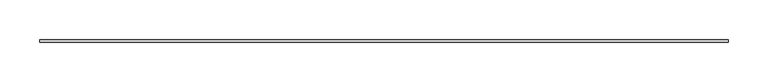
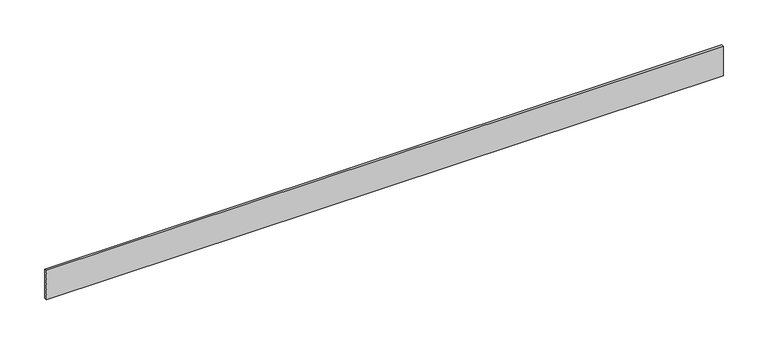
"""IFC4 building model written with IfcOpenShell, lengths in millimetres: proxy geometry, Generic Models 3:Generic Models 1:3:Generic Models 1:3 : Generic Models 3:Generic Models 1:300625:336034:Generic Models 1:3:Generic Models 1:3 : Generic Models 3:Generic Models 1:300625:336034 : Generic Models 3:Generic Models 1:3:Generic Models 1:3 : Generic Models 3:Generic Models 1:300625:336034:4 : Generic Models 3:Generic Models 1:3:Generic Models 1:3 : Generic Models 3:Generic Models 1:300625:336034:Generic Models 1:3:Generic Models 1:3 : Generic Models 3:Generic Models 1:300625:336034 : Generic Models 3:Generic Models 1:3:Generic Models 1:3 : Generic Models 3:Generic Models 1:300625:336034:301191."""

import ifcopenshell
import ifcopenshell.guid

model = None  # the IFC model being written
_history = None  # IfcOwnerHistory: only IFC2X3 demands one
_inside = {}  # id of a spatial element -> (the spatial element, [elements in it])
_under = {}  # id of a project, library or spatial element -> (it, [spatial elements below it])
_declared = {}  # id of a project -> (the project, [libraries it declares])
_typed = {}  # id of a type object -> (the type object, [elements of that type])
_made_of = {}  # id of a material, layer set ... -> (it, [elements and type objects made of it])


def new_model(schema):
    """Start an empty IFC model of exactly this schema.

    Asked for "IFC4X3", IfcOpenShell would pick the latest addendum, in which some entities
    have other attributes; the version numbers below select the first issue.
    IFC2X3 requires an IfcOwnerHistory on every rooted entity: one is made here for all.
    """
    global model, _history
    if schema == "IFC4X3":
        model = ifcopenshell.file(schema_version=(4, 3, 0, 0))
    else:
        model = ifcopenshell.file(schema=schema)
    _inside.clear()
    _under.clear()
    _declared.clear()
    _typed.clear()
    _made_of.clear()
    _history = None
    if model.schema == "IFC2X3":
        org = make("IfcOrganization", Name="unknown")
        user = make(
            "IfcPersonAndOrganization",
            ThePerson=make("IfcPerson", FamilyName="unknown"),
            TheOrganization=org,
        )
        app = make(
            "IfcApplication",
            ApplicationDeveloper=org,
            Version="unknown",
            ApplicationFullName="unknown",
            ApplicationIdentifier="unknown",
        )
        _history = make(
            "IfcOwnerHistory",
            OwningUser=user,
            OwningApplication=app,
            ChangeAction="ADDED",
            CreationDate=0,
        )
    return model


def make(cls, **values):
    """One entity of the class cls with the attributes given. An attribute that is None is left unset."""
    return model.create_entity(
        cls, **{name: value for name, value in values.items() if value is not None}
    )


def rooted(cls, **values):
    """An entity with a GlobalId (a new one), such as an element, a storey or a relation."""
    return make(cls, GlobalId=ifcopenshell.guid.new(), OwnerHistory=_history, **values)


def si_unit(unit_type, name, prefix=None):
    """IfcSIUnit, for example si_unit("LENGTHUNIT", "METRE", prefix="MILLI")."""
    return make("IfcSIUnit", UnitType=unit_type, Prefix=prefix, Name=name)


def assignment(units):
    """IfcUnitAssignment: the units of a project."""
    return None if units is None else make("IfcUnitAssignment", Units=units)


def point(xyz):
    """IfcCartesianPoint."""
    return None if xyz is None else make("IfcCartesianPoint", Coordinates=xyz)


def direction(xyz):
    """IfcDirection."""
    return None if xyz is None else make("IfcDirection", DirectionRatios=xyz)


def frame(location, z_axis=None, x_axis=None):
    """IfcAxis2Placement3D, a coordinate frame: its origin and axes. An axis left out is left unset."""
    return make(
        "IfcAxis2Placement3D",
        Location=point(location),
        Axis=direction(z_axis),
        RefDirection=direction(x_axis),
    )


def origin():
    """The frame at (0, 0, 0) with its axes left unset."""
    return frame((0.0, 0.0, 0.0))


def place(relative_to, where):
    """IfcLocalPlacement: puts the frame where relative to a parent placement (None: the world)."""
    return make(
        "IfcLocalPlacement", PlacementRelTo=relative_to, RelativePlacement=where
    )


def context(
    kind, dimensions, precision=None, world=None, true_north=None, identifier=None
):
    """IfcGeometricRepresentationContext, for example the 3D "Model" context."""
    return make(
        "IfcGeometricRepresentationContext",
        ContextIdentifier=identifier,
        ContextType=kind,
        CoordinateSpaceDimension=dimensions,
        Precision=precision,
        WorldCoordinateSystem=world,
        TrueNorth=true_north,
    )


def project(units=None, contexts=None):
    """IfcProject with its units and contexts."""
    return rooted(
        "IfcProject",
        Name="project",
        RepresentationContexts=contexts,
        UnitsInContext=assignment(units),
    )


def spatial(cls, under=None, at=None, **own):
    """A site, building, storey or space (cls), placed at a placement, below another one or the project."""
    s = rooted(cls, ObjectPlacement=at, **own)
    if under is not None:
        _under.setdefault(under.id(), (under, []))[1].append(s)
    return s


def polyline(points):
    """IfcPolyline through the points."""
    return make("IfcPolyline", Points=[point(p) for p in points])


def outline(outer, holes=None, kind="AREA"):
    """IfcArbitraryClosedProfileDef: a profile drawn as a closed curve; with holes, ...WithVoids."""
    if holes is None:
        return make("IfcArbitraryClosedProfileDef", ProfileType=kind, OuterCurve=outer)
    return make(
        "IfcArbitraryProfileDefWithVoids",
        ProfileType=kind,
        OuterCurve=outer,
        InnerCurves=holes,
    )


def extrude(swept, where, along, depth):
    """IfcExtrudedAreaSolid: the profile swept, set in the frame where, extruded along a direction by depth."""
    return make(
        "IfcExtrudedAreaSolid",
        SweptArea=swept,
        Position=where,
        ExtrudedDirection=direction(along),
        Depth=depth,
    )


def shape(context_of_items, identifier, shape_type, items):
    """IfcShapeRepresentation: the items that make up one representation, for example the "Body"."""
    return make(
        "IfcShapeRepresentation",
        ContextOfItems=context_of_items,
        RepresentationIdentifier=identifier,
        RepresentationType=shape_type,
        Items=items,
    )


def source(mapping_origin, context_of_items, identifier, shape_type, items):
    """IfcRepresentationMap: a shape defined once, which mapped items show again and again."""
    return make(
        "IfcRepresentationMap",
        MappingOrigin=mapping_origin,
        MappedRepresentation=shape(context_of_items, identifier, shape_type, items),
    )


def transform(
    local_origin,
    x_axis=None,
    y_axis=None,
    z_axis=None,
    scale=None,
    scale2=None,
    scale3=None,
    uniform=True,
):
    """IfcCartesianTransformationOperator3D, or its non-uniform kind. x_axis, y_axis, z_axis: its Axis1, 2, 3."""
    if uniform:
        return make(
            "IfcCartesianTransformationOperator3D",
            Axis1=direction(x_axis),
            Axis2=direction(y_axis),
            LocalOrigin=point(local_origin),
            Scale=scale,
            Axis3=direction(z_axis),
        )
    return make(
        "IfcCartesianTransformationOperator3DnonUniform",
        Axis1=direction(x_axis),
        Axis2=direction(y_axis),
        LocalOrigin=point(local_origin),
        Scale=scale,
        Axis3=direction(z_axis),
        Scale2=scale2,
        Scale3=scale3,
    )


def mapped(mapping_source, mapping_target):
    """IfcMappedItem: shows the shape of a source again, moved by a transform."""
    return make(
        "IfcMappedItem", MappingSource=mapping_source, MappingTarget=mapping_target
    )


def made_of(thing, what):
    """Note that an element or type object is made of a material, layer set ...; save() writes the relation."""
    if what is not None:
        _made_of.setdefault(what.id(), (what, []))[1].append(thing)
    return thing


def element(
    cls,
    number,
    at=None,
    inside=None,
    cuts=None,
    type_object=None,
    material=None,
    context=None,
    identifier="Body",
    shape_type=None,
    held_by="IfcProductDefinitionShape",
    body=None,
    shapes=None,
    **own,
):
    """One element of the class cls, such as IfcWall. Its Tag is "e" and its number.

    at: its placement. inside: the storey or other place that contains it. cuts: it is an
    opening in that element (IfcRelVoidsElement). A single representation is given by context,
    identifier, shape_type and body (its items); several are given by shapes. held_by: the class
    of the entity that holds the representations. save() writes the other relations.
    """
    e = rooted(cls, Tag="e%d" % number, ObjectPlacement=at, **own)
    if body is not None:
        shapes = [shape(context, identifier, shape_type, body)]
    if shapes is not None:
        e.Representation = make(held_by, Representations=shapes)
    if inside is not None:
        _inside.setdefault(inside.id(), (inside, []))[1].append(e)
    if cuts is not None:
        rooted(
            "IfcRelVoidsElement", RelatingBuildingElement=cuts, RelatedOpeningElement=e
        )
    if type_object is not None:
        _typed.setdefault(type_object.id(), (type_object, []))[1].append(e)
    return made_of(e, material)


def aggregate(whole, parts):
    """IfcRelAggregates: a whole, such as a stair, and the parts it consists of."""
    return rooted("IfcRelAggregates", RelatingObject=whole, RelatedObjects=parts)


def save(model, path):
    """Write the relations noted so far, then the file.

    IfcRelAggregates (storeys below a building ...), IfcRelContainedInSpatialStructure (elements
    in a storey), IfcRelDefinesByType, IfcRelAssociatesMaterial and IfcRelDeclares: one each for
    every whole, place, type object, material and project.
    """
    for whole, parts in _under.values():
        aggregate(whole, parts)
    for where, things in _inside.values():
        rooted(
            "IfcRelContainedInSpatialStructure",
            RelatedElements=things,
            RelatingStructure=where,
        )
    for kind, things in _typed.values():
        rooted("IfcRelDefinesByType", RelatedObjects=things, RelatingType=kind)
    for what, things in _made_of.values():
        rooted("IfcRelAssociatesMaterial", RelatedObjects=things, RelatingMaterial=what)
    for by, libraries in _declared.values():
        rooted("IfcRelDeclares", RelatingContext=by, RelatedDefinitions=libraries)
    model.write(path)


def generic_models_05a2607f(model_context):
    return source(origin(), model_context, "Body", "SweptSolid", [
        extrude(outline(polyline([(570395.4867239, -579000.6913841), (570395.4867239, -579003.8663841), (569527.1242239, -579003.8663841), (569527.1242239, -579000.6913841), (570395.4867239, -579000.6913841)])), frame((0.0, 0.0, 2446.5359375), z_axis=(0.0, 0.0, 1.0), x_axis=(1.0, 0.0, 0.0)), (0.0, 0.0, 1.0), 39.74694),
    ])


if __name__ == "__main__":
    model = new_model("IFC4")
    model_context = context("Model", 3, world=origin())
    ifc_project = project(units=[si_unit("LENGTHUNIT", "METRE", prefix="MILLI")], contexts=[model_context])
    site = spatial("IfcSite", under=ifc_project)
    building = spatial("IfcBuilding", under=site)
    placement = place(None, origin())
    generic_models_shape = generic_models_05a2607f(model_context)
    element("IfcBuildingElementProxy", 1, Name="Generic Models 3:Generic Models 1:3:Generic Models 1:3 : Generic Models 3:Generic Models 1:300625:336034:Generic Models 1:3:Generic Models 1:3 : Generic Models 3:Generic Models 1:300625:336034 : Generic Models 3:Generic Models 1:3:Generic Models 1:3 : Generic Models 3:Generic Models 1:300625:336034:4 : Generic Models 3:Generic Models 1:3:Generic Models 1:3 : Generic Models 3:Generic Models 1:300625:336034:Generic Models 1:3:Generic Models 1:3 : Generic Models 3:Generic Models 1:300625:336034 : Generic Models 3:Generic Models 1:3:Generic Models 1:3 : Generic Models 3:Generic Models 1:300625:336034:301191", ObjectType="Generic Models 3:Generic Models 1:3:Generic Models 1:3 : Generic Models 3:Generic Models 1:300625:336034:Generic Models 1:3:Generic Models 1:3 : Generic Models 3:Generic Models 1:300625:336034 : Generic Models 3:Generic Models 1:3:Generic Models 1:3 : Generic Models 3:Generic Models 1:300625:336034:4 : Generic Models 3:Generic Models 1:3:Generic Models 1:3 : Generic Models 3:Generic Models 1:300625:336034:Generic Models 1:3:Generic Models 1:3 : Generic Models 3:Generic Models 1:300625:336034 : Generic Models 3:Generic Models 1:3:Generic Models 1:3 : Generic Models 3:Generic Models 1:300625:336034:301191", at=placement, inside=building, context=model_context, shape_type="MappedRepresentation", body=[
        mapped(generic_models_shape, transform((0.0, 0.0, 0.0), x_axis=(1.0, 0.0, 0.0), y_axis=(0.0, 1.0, 0.0), z_axis=(0.0, 0.0, 1.0))),
    ])
    save(model, "model.ifc")

# Revit data of these elements
# Type "Generic Models 3:Generic Models 1:3:Generic Models 1:3 : Generic Models 3:Generic Models 1:300625:336034:Generic Models 1:3:Generic Models 1:3 : Generic Models 3:Generic Models 1:300625:336034 : Generic Models 3:Generic Models 1:3:Generic Models 1:3 : Generic Models 3:Generic Models 1:300625:336034:4 : Generic Models 3:Generic Models 1:3:Generic Models 1:3 : Generic Models 3:Generic Models 1:300625:336034:Generic Models 1:3:Generic Models 1:3 : Generic Models 3:Generic Models 1:300625:336034 : Generic Models 3:Generic Models 1:3:Generic Models 1:3 : Generic Models 3:Generic Models 1:300625:336034:301191"
#   NameOverride = "Generic Models 3:Generic Models 1:3:Generic Models 1:3 : Generic Models 3:Generic Models 1:300625:336034:Generic Models 1:3:Generic Models 1:3 : Generic Models 3:Generic Models 1:300625:336034 : Generic Models 3:Generic Models 1:3:Generic Models 1:3 : Generic Models 3:Generic Models 1:300625:336034:301191"
#   ObjectTypeOverride = "Generic Models 1:3:Generic Models 1:3 : Generic Models 3:Generic Models 1:300625:336034 : Generic Models 3:Generic Models 1:3:Generic Models 1:3 : Generic Models 3:Generic Models 1:300625:336034"
#   Reference = "Generic Models 1"
#   Tag = "301191"
# Element 1 (IfcBuildingElementProxy, "Generic Models 3:Generic Models 1:3:Generic Models 1:3 : Generic Models 3:Generic Models 1:300625:336034:Generic Models 1:3:Generic Models 1:3 : Generic Models 3:Generic Models 1:300625:336034 : Generic Models 3:Generic Models 1:3:Generic Models 1:3 : Generic Models 3:Generic Models 1:300625:336034:4 : Generic Models 3:Generic Models 1:3:Generic Models 1:3 : Generic Models 3:Generic Models 1:300625:336034:Generic Models 1:3:Generic Models 1:3 : Generic Models 3:Generic Models 1:300625:336034 : Generic Models 3:Generic Models 1:3:Generic Models 1:3 : Generic Models 3:Generic Models 1:300625:336034:301191")
#   Materials on its faces: "COMPRESSIBE THERMAL GASKET SANDWICHED BETWEEN METAL COMPONENTS"
# Materials
#   "COMPRESSIBE THERMAL GASKET SANDWICHED BETWEEN METAL COMPONENTS": class "Unassigned", colour RGB 58 208 21, transparency 0, Cost = 0
